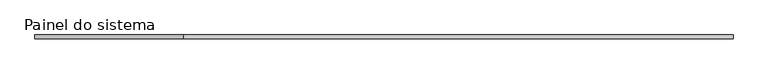
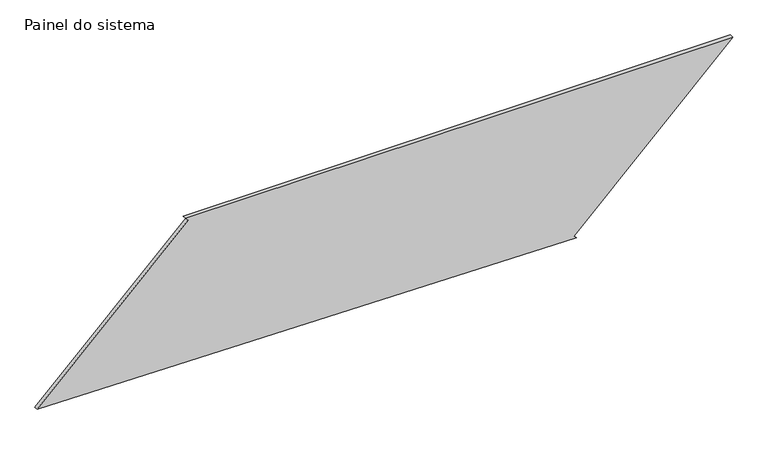
"""IFC4 building model written with IfcOpenShell, lengths in millimetres: plate geometry, Painel do sistema : Envidraçado."""

from ifc_helpers import new_model, si_unit, frame, origin, place, context, project, spatial, polyline, outline, extrude, source, transform, mapped, element, save


def painel_do_sistema_17f6bbd4(model_context):
    return source(origin(), model_context, "Body", "SweptSolid", [
        extrude(outline(polyline([(0.0, 1277.457994), (17.9061609, 1260.0118081), (1051.1646865, 2320.512574), (1051.1646865, -1330.1835737), (1033.2585256, -1312.7373879), (51.3711603, -2320.512574), (0.0, 1277.457994)])), frame((0.0, 24.5, 0.0), z_axis=(0.0, 1.0, 0.0), x_axis=(0.0, 0.0, 1.0)), (0.0, 0.0, 1.0), 25.0),
    ])


if __name__ == "__main__":
    model = new_model("IFC4")
    model_context = context("Model", 3, world=origin())
    ifc_project = project(units=[si_unit("LENGTHUNIT", "METRE", prefix="MILLI")], contexts=[model_context])
    site = spatial("IfcSite", under=ifc_project)
    building = spatial("IfcBuilding", under=site)
    placement = place(None, origin())
    painel_do_sistema_shape = painel_do_sistema_17f6bbd4(model_context)
    element("IfcPlate", 1, ObjectType="Painel do sistema : Envidraçado", at=placement, inside=building, context=model_context, shape_type="MappedRepresentation", body=[
        mapped(painel_do_sistema_shape, transform((0.0, 0.0, 0.0), x_axis=(1.0, 0.0, 0.0), y_axis=(0.0, 1.0, 0.0), z_axis=(0.0, 0.0, 1.0))),
    ])
    save(model, "model.ifc")

# Revit data of these elements
# Type "Painel do sistema : Envidraçado"
#   Construction Type Id = "GSP4R"
#   Analytic Construction = "Vidraça única Pilkington 1/8 pol"
#   Visual Light Transmittance = 0.9
#   Solar Heat Gain Coefficient = 0.86
#   Heat Transfer Coefficient (U) = 6.7069 W/(m²·K)
# Element 1 (IfcPlate, "Painel do sistema : Envidraçado")
#   Materials on its faces: "Vidro"
# Materials
#   "Vidro": class "Vidro", colour RGB 0 128 192, transparency 0.9, Description = "Vidro de sílica", Cost = 0
